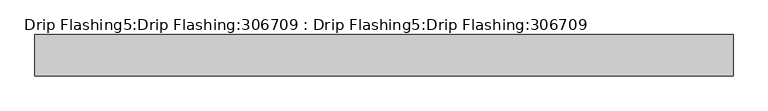
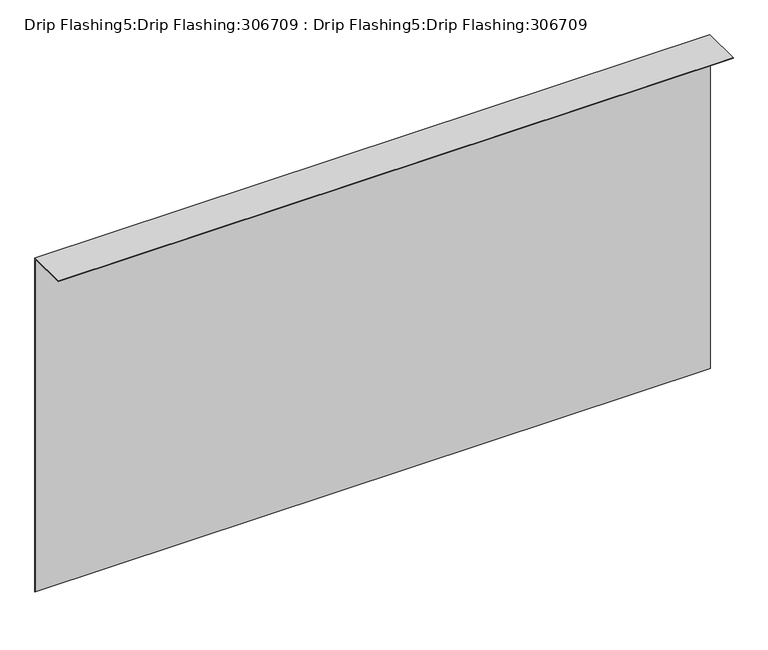
"""IFC4 building model written with IfcOpenShell, lengths in millimetres: proxy geometry, Drip Flashing5:Drip Flashing:306709 : Drip Flashing5:Drip Flashing:306709."""

from ifc_helpers import new_model, si_unit, frame, origin, place, context, project, spatial, polyline, outline, extrude, source, transform, mapped, element, save


def drip_flashing5_drip_flashing_306709_drip_flashing5_drip_05b6835c(model_context):
    return source(origin(), model_context, "Body", "SweptSolid", [
        extrude(outline(polyline([(10021.1238058, 36556.696), (10021.1238058, 37600.3015275), (9903.7868933, 37600.3015275), (9903.7868933, 37601.8015275), (10022.6238058, 37601.8015275), (10022.6238058, 36556.696), (10021.1238058, 36556.696)])), frame((-4455.0628198, 0.0, 0.0), z_axis=(1.0, 0.0, 0.0), x_axis=(0.0, 1.0, 0.0)), (0.0, 0.0, 1.0), 1999.85),
    ])


if __name__ == "__main__":
    model = new_model("IFC4")
    model_context = context("Model", 3, world=origin())
    ifc_project = project(units=[si_unit("LENGTHUNIT", "METRE", prefix="MILLI")], contexts=[model_context])
    site = spatial("IfcSite", under=ifc_project)
    building = spatial("IfcBuilding", under=site)
    placement = place(None, origin())
    drip_flashing5_drip_flashing_306709_drip_flashing5_drip_shape = drip_flashing5_drip_flashing_306709_drip_flashing5_drip_05b6835c(model_context)
    element("IfcBuildingElementProxy", 1, Name="Drip Flashing5:Drip Flashing:306709 : Drip Flashing5:Drip Flashing:306709", ObjectType="Drip Flashing5:Drip Flashing:306709 : Drip Flashing5:Drip Flashing:306709", at=placement, inside=building, context=model_context, shape_type="MappedRepresentation", body=[
        mapped(drip_flashing5_drip_flashing_306709_drip_flashing5_drip_shape, transform((0.0, 0.0, 0.0), x_axis=(1.0, 0.0, 0.0), y_axis=(0.0, 1.0, 0.0), z_axis=(0.0, 0.0, 1.0))),
    ])
    save(model, "model.ifc")

# Revit data of these elements
# Type "Drip Flashing5:Drip Flashing:306709 : Drip Flashing5:Drip Flashing:306709"
#   NameOverride = "Drip Flashing5:Drip Flashing:306709"
#   ObjectTypeOverride = "Drip Flashing5:Drip Flashing"
#   Reference = "Drip Flashing"
#   Category = "Generic Models"
#   Tag = "306709"
# Element 1 (IfcBuildingElementProxy, "Drip Flashing5:Drip Flashing:306709 : Drip Flashing5:Drip Flashing:306709")
#   Materials on its faces: "(2) LAYERS OF ICE & WATER SHIELD (BITUTHANE) UNDER STUCCO"
# Materials
#   "(2) LAYERS OF ICE & WATER SHIELD (BITUTHANE) UNDER STUCCO": class "Unassigned", colour RGB 186 255 159, transparency 0, Cost = 0
